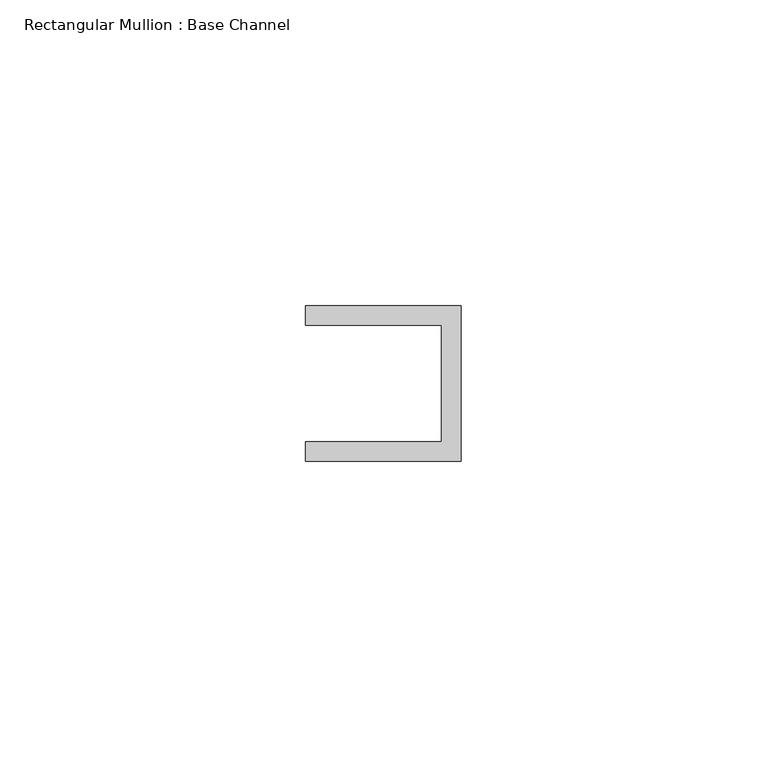
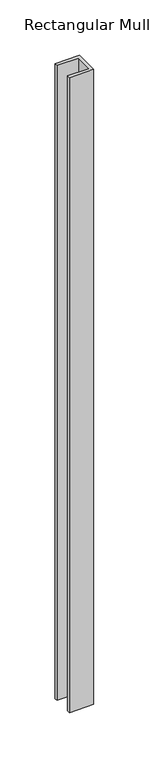
"""IFC4 building model written with IfcOpenShell, lengths in millimetres: member geometry, Rectangular Mullion : Base Channel."""

from ifc_helpers import new_model, si_unit, frame, origin, place, context, project, spatial, polyline, outline, extrude, source, transform, mapped, element, save


def rectangular_mullion_base_channel_d9767c24(model_context):
    return source(origin(), model_context, "Body", "SweptSolid", [
        extrude(outline(polyline([(0.0, -12.7), (-25.4, -12.7), (-25.4, -9.525), (-3.175, -9.525), (-3.175, 9.525), (-25.4, 9.525), (-25.4, 12.7), (0.0, 12.7), (0.0, -12.7)])), frame((0.0, 0.0, -698.5), z_axis=(0.0, 0.0, 1.0), x_axis=(1.0, 0.0, 0.0)), (0.0, 0.0, 1.0), 698.5),
    ])


if __name__ == "__main__":
    model = new_model("IFC4")
    model_context = context("Model", 3, world=origin())
    ifc_project = project(units=[si_unit("LENGTHUNIT", "METRE", prefix="MILLI")], contexts=[model_context])
    site = spatial("IfcSite", under=ifc_project)
    building = spatial("IfcBuilding", under=site)
    placement = place(None, origin())
    rectangular_mullion_base_channel_shape = rectangular_mullion_base_channel_d9767c24(model_context)
    element("IfcMember", 1, ObjectType="Rectangular Mullion : Base Channel", at=placement, inside=building, context=model_context, shape_type="MappedRepresentation", body=[
        mapped(rectangular_mullion_base_channel_shape, transform((0.0, 0.0, 0.0), x_axis=(1.0, 0.0, 0.0), y_axis=(0.0, 1.0, 0.0), z_axis=(0.0, 0.0, 1.0))),
    ])
    save(model, "model.ifc")

# Revit data of these elements
# Type "Rectangular Mullion : Base Channel"
#   built-in parameter 1007322 = 0.0833333 (stored number, unit not read)
#   built-in parameter 1007321 = 0.0416667 (stored number, unit not read)
#   built-in parameter 1007320 = -0.03125 (stored number, unit not read)
# Element 1 (IfcMember, "Rectangular Mullion : Base Channel")
#   Materials on its faces: "ALUM"
# Materials
#   "ALUM": class "Generic", colour RGB 157 157 157, transparency 0, Cost = 0
